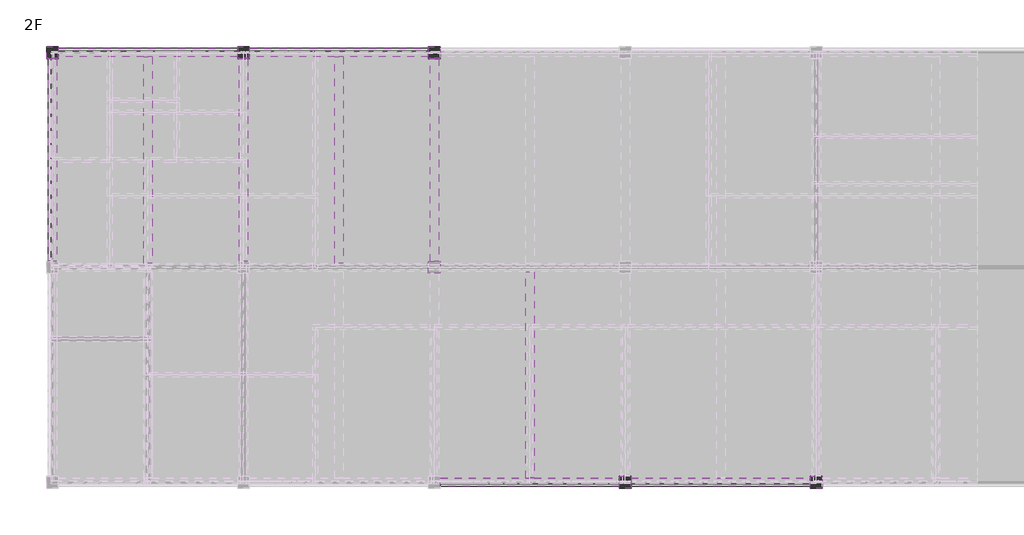
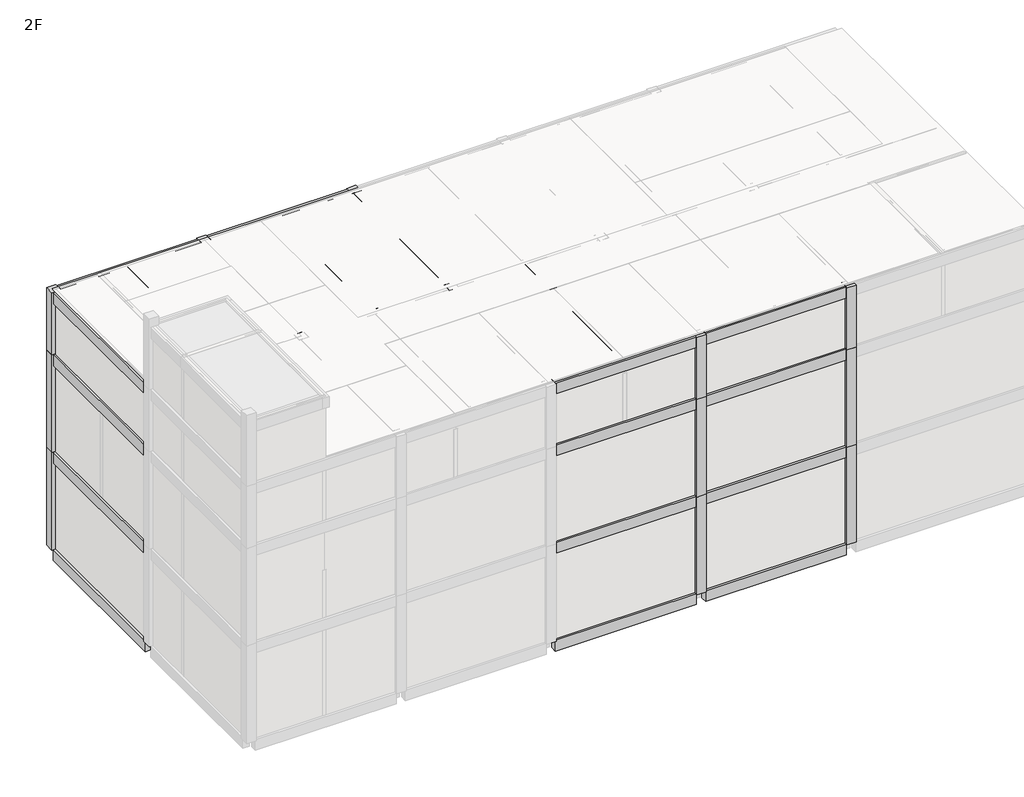
# One storey, part 5 of 7: 40 beams, 17 columns.
# Revit data of these elements (continued)
# Room at (47459.652, 166923.861) mm, phase "New Construction", upper offset 2700 mm, lower offset 0 mm (continued)
#   Name = "Staircase"
#   Interior Finish = "IW5..N/A..N/A,,WK3..N/A,,FL2..N/A,,CL1..N/A"
#   Exterior Finish = "N/A..N/A,,EW2..N/A..N/A"
# Room at (82459.652, 177423.861) mm, phase "New Construction", upper offset 2700 mm, lower offset 0 mm
#   Department = "AR"
#   Base Finish = "WK3"
#   Ceiling Finish = "CL3"
#   Wall Finish = "IW5"
#   Floor Finish = "FL2"
#   Number = "3.12"
#   Name = "Corridor"
#   Interior Finish = "IW5..N/A..N/A,,WK3..N/A,,FL2..N/A,,CL3..N/A"
#   Exterior Finish = "N/A..N/A,,EW2..N/A..N/A"
# Room at (51459.652, 170673.861) mm, phase "New Construction", upper offset 2700 mm, lower offset 0 mm
#   Department = "AR"
#   Base Finish = "WK3"
#   Ceiling Finish = "CL3"
#   Wall Finish = "IW5"
#   Floor Finish = "FL2"
#   Number = "3.13"
#   Name = "Corridor"
#   Interior Finish = "IW5..N/A..N/A,,WK3..N/A,,FL2..N/A,,CL3..N/A"
#   Exterior Finish = "N/A..N/A,,EW2..N/A..N/A"
# Room at (63459.652, 167173.861) mm, phase "New Construction", upper offset 2700 mm, lower offset 0 mm
#   Department = "AR"
#   Base Finish = "WK3"
#   Ceiling Finish = "CL3"
#   Wall Finish = "IW5"
#   Floor Finish = "FL2"
#   Number = "4.0"
#   Name = "Manager Office-1"
#   Interior Finish = "IW5..N/A..N/A,,WK3..N/A,,FL2..N/A,,CL3..N/A"
#   Exterior Finish = "RF1..N/A,,EW1..N/A..N/A"
# Room at (67459.652, 167173.861) mm, phase "New Construction", upper offset 2700 mm, lower offset 0 mm
#   Department = "AR"
#   Base Finish = "WK3"
#   Ceiling Finish = "CL3"
#   Wall Finish = "IW5"
#   Floor Finish = "FL2"
#   Number = "4.1"
#   Name = "Manager Office-2"
#   Interior Finish = "IW5..N/A..N/A,,WK3..N/A,,FL2..N/A,,CL3..N/A"
#   Exterior Finish = "RF1..N/A,,EW1..N/A..N/A"
# Room at (78709.652, 178923.861) mm, phase "New Construction", upper offset 2700 mm, lower offset 0 mm
#   Department = "AR"
#   Base Finish = "WK3"
#   Ceiling Finish = "CL3"
#   Wall Finish = "IW5"
#   Floor Finish = "FL2"
#   Number = "4.2"
#   Name = "Meeting Room-1"
#   Interior Finish = "IW5..N/A..N/A,,WK3..N/A,,FL2..N/A,,CL3..N/A"
#   Exterior Finish = "RF1..N/A,,EW1..EW2..N/A"
# Room at (73459.652, 167173.861) mm, phase "New Construction", upper offset 2700 mm, lower offset 0 mm
#   Department = "AR"
#   Base Finish = "WK3"
#   Ceiling Finish = "CL3"
#   Wall Finish = "IW5"
#   Floor Finish = "FL2"
#   Number = "4.3"
#   Name = "Meeting Room-2"
#   Interior Finish = "IW5..N/A..N/A,,WK3..N/A,,FL2..N/A,,CL3..N/A"
#   Exterior Finish = "RF1..N/A,,EW1..N/A..N/A"
# Room at (64709.652, 177423.861) mm, phase "New Construction", upper offset 2700 mm, lower offset 0 mm
#   Department = "HV"
#   Base Finish = "WK3"
#   Ceiling Finish = "CL3"
#   Wall Finish = "IW5"
#   Floor Finish = "FL2"
#   Number = "4.4"
#   Name = "Open Office"
#   Interior Finish = "IW5..N/A..N/A,,WK3..N/A,,FL2..N/A,,CL3..N/A"
#   Exterior Finish = "RF1..N/A,,EW1..N/A..N/A"
# Room at (54959.652, 178923.861) mm, phase "New Construction", upper offset 2700 mm, lower offset 0 mm
#   Department = "AR"
#   Base Finish = "WK3"
#   Ceiling Finish = "CL3"
#   Wall Finish = "IW5"
#   Floor Finish = "FL2"
#   Number = "4.12"
#   Name = "Locker(M)"
#   Interior Finish = "IW5..N/A..N/A,,WK3..N/A,,FL2..N/A,,CL3..N/A"
#   Exterior Finish = "RF1..N/A,,EW1..N/A..N/A"
# Room at (50659.652, 174423.861) mm, phase "New Construction", upper offset 2700 mm, lower offset 0 mm
#   Department = "AR"
#   Base Finish = ""
#   Ceiling Finish = "CL4"
#   Wall Finish = "IW3"
#   Floor Finish = "FL3"
#   Number = "4.13"
#   Name = "Toilet(F)"
#   Interior Finish = "IW3..N/A..N/A,,N/A..N/A,,FL3..N/A,,CL4..N/A"
#   Exterior Finish = "RF1..N/A,,N/A..N/A..N/A"
# Room at (46659.652, 177423.861) mm, phase "New Construction", upper offset 3500 mm, lower offset 0 mm
#   Department = "PATHV3"
#   Base Finish = ""
#   Ceiling Finish = ""
#   Wall Finish = ""
#   Floor Finish = ""
#   Number = "4.14"
#   Name = "Duct Shaft"
#   Interior Finish = "N/A..N/A..N/A,,N/A..N/A,,N/A..N/A,,N/A..N/A"
#   Exterior Finish = "RF1..N/A,,EW2..N/A..N/A"
# Room at (47459.652, 171423.861) mm, phase "New Construction", upper offset 3500 mm, lower offset 0 mm
#   Department = "PATHV2"
#   Base Finish = ""
#   Ceiling Finish = ""
#   Wall Finish = ""
#   Floor Finish = ""
#   Number = "4.15"
#   Name = "Elevator"
#   Interior Finish = "N/A..N/A..N/A,,N/A..N/A,,N/A..N/A,,N/A..N/A"
#   Exterior Finish = "N/A..N/A,,EW2..N/A..N/A"
# Room at (47459.652, 166923.861) mm, phase "New Construction", upper offset 3500 mm, lower offset 0 mm
#   Department = "PATHV1"
#   Base Finish = ""
#   Ceiling Finish = "CL1"
#   Wall Finish = "IW5"
#   Floor Finish = "FL2"
#   Number = "4.16"
#   Name = "Staircase"
#   Interior Finish = "IW5..N/A..N/A,,N/A..N/A,,FL2..N/A,,CL1..N/A"
#   Exterior Finish = "N/A..N/A,,EW2..N/A..N/A"
# Room at (61397.694, 171673.861) mm, phase "New Construction", upper offset 2700 mm, lower offset 0 mm
#   Department = "AR"
#   Base Finish = "WK3"
#   Ceiling Finish = "CL3"
#   Wall Finish = "IW5"
#   Floor Finish = "FL2"
#   Number = "4.17"
#   Name = "Corridor"
#   Interior Finish = "IW5..N/A..N/A,,WK3..N/A,,FL2..N/A,,CL3..N/A"
#   Exterior Finish = "RF1..N/A,,EW2..N/A..N/A"
# Room at (47459.652, 171423.861) mm, phase "New Construction", upper offset 3500 mm, lower offset 0 mm
#   Department = "PATHV2"
#   Base Finish = ""
#   Ceiling Finish = ""
#   Wall Finish = ""
#   Floor Finish = ""
#   Number = "5.0"
#   Name = "Elevator"
#   Interior Finish = "N/A..N/A..N/A,,N/A..N/A,,N/A..N/A,,N/A..N/A"
#   Exterior Finish = "RF1..N/A,,EW2..EW1..N/A"
# Room at (47459.652, 166923.861) mm, phase "New Construction", upper offset 3500 mm, lower offset 0 mm
#   Department = "PATHV1"
#   Base Finish = "WK3"
#   Ceiling Finish = "CL1"
#   Wall Finish = "IW5"
#   Floor Finish = "FL2"
#   Number = "5.1"
#   Name = "Staircase"
#   Interior Finish = "IW5..N/A..N/A,,WK3..N/A,,FL2..N/A,,CL1..N/A"
#   Exterior Finish = "RF1..N/A,,EW2..EW1..N/A"
